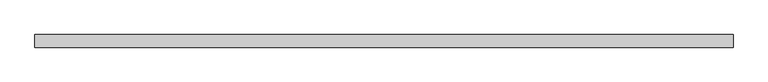
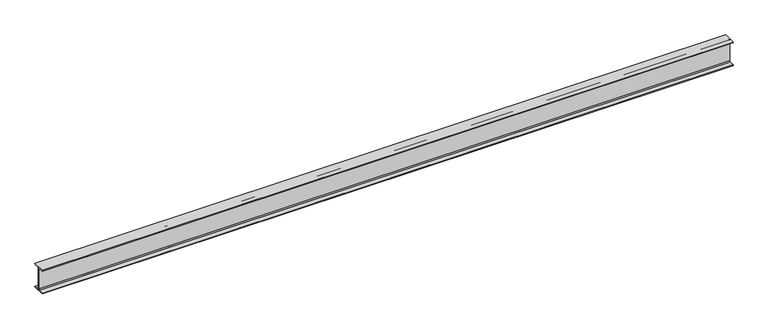
"""IFC4 building model written with IfcOpenShell, lengths in millimetres: beam geometry, 0912_Steel Framing_H-KSD3502 : H_SB_ASB_H-350x175x7x11."""

from ifc_helpers import new_model, si_unit, point, frame, frame_2d, origin, place, context, project, spatial, polyline, circle_curve, trimmed, segment, composite_curve, outline, extrude, source, transform, mapped, element, save


def beam_b0d276df(model_context):
    return source(origin(), model_context, "Body", "SweptSolid", [
        extrude(outline(composite_curve([segment(polyline([(87.5, -164.0), (87.5, -175.0), (-87.5, -175.0), (-87.5, -164.0), (-17.5, -164.0)]), True, "CONTINUOUS"), segment(trimmed(circle_curve(frame_2d((-17.5, -150.0)), 14.0), [point((-17.5, -164.0))], [point((-3.5, -150.0))], True, "CARTESIAN"), True, "CONTINUOUS"), segment(polyline([(-3.5, -150.0), (-3.5, 150.0)]), True, "CONTINUOUS"), segment(trimmed(circle_curve(frame_2d((-17.5, 150.0)), 14.0), [point((-3.5, 150.0))], [point((-17.5, 164.0))], True, "CARTESIAN"), True, "CONTINUOUS"), segment(polyline([(-17.5, 164.0), (-87.5, 164.0), (-87.5, 175.0), (87.5, 175.0), (87.5, 164.0), (17.5, 164.0)]), True, "CONTINUOUS"), segment(trimmed(circle_curve(frame_2d((17.5, 150.0)), 14.0), [point((17.5, 164.0))], [point((3.5, 150.0))], True, "CARTESIAN"), True, "CONTINUOUS"), segment(polyline([(3.5, 150.0), (3.5, -150.0)]), True, "CONTINUOUS"), segment(trimmed(circle_curve(frame_2d((17.5, -150.0)), 14.0), [point((3.5, -150.0))], [point((17.5, -164.0))], True, "CARTESIAN"), True, "CONTINUOUS"), segment(polyline([(17.5, -164.0), (87.5, -164.0)]), True, "CONTINUOUS")], self_intersect=False)), frame((-4837.3, 0.0, 0.0), z_axis=(1.0, 0.0, 0.0), x_axis=(0.0, 1.0, 0.0)), (0.0, 0.0, 1.0), 9699.6),
    ])


if __name__ == "__main__":
    model = new_model("IFC4")
    model_context = context("Model", 3, world=origin())
    ifc_project = project(units=[si_unit("LENGTHUNIT", "METRE", prefix="MILLI")], contexts=[model_context])
    site = spatial("IfcSite", under=ifc_project)
    building = spatial("IfcBuilding", under=site)
    placement = place(None, origin())
    beam_shape = beam_b0d276df(model_context)
    element("IfcBeam", 1, ObjectType="0912_Steel Framing_H-KSD3502 : H_SB_ASB_H-350x175x7x11", at=placement, inside=building, context=model_context, shape_type="MappedRepresentation", body=[
        mapped(beam_shape, transform((0.0, 0.0, 0.0), x_axis=(1.0, 0.0, 0.0), y_axis=(0.0, 1.0, 0.0), z_axis=(0.0, 0.0, 1.0))),
    ])
    save(model, "model.ifc")

# Revit data of these elements
# Type "0912_Steel Framing_H-KSD3502 : H_SB_ASB_H-350x175x7x11"
#   H_WM Code_1 = "S01AA002-00001 | Main Steel Structure Fabrication Work | Shelter/Building | Medium Steel - Standard (90KG/M>Weight≥30KG/M) | Material: (   )"
#   H_WM Code_2 = "S03AA028-00001 | Main Steel Structure Erection Work | Shelter/Building | Medium Steel (90KG/M>Weight≥30KG/M) | Material: (   )"
#   H_WM Code_3 = "S01AA010-00001 | Main Steel Structure Fabrication Work | Shelter/Building | Steel Painting/Coating | for Non-Fireproofed Steel Surface, Surface Preparation, Primer, Second & Final Coat | Material: (   )"
#   H_Q'ty Cal Type Tag = "SB-Q2"
#   Width = 17.5 cm
#   Web Thickness = 0.7 cm
#   Web Fillet = 1.4 cm
#   Warping Constant = 282000.0 cm⁶
#   W = 0
#   Torsional Moment of Inertia = 19.4042 cm⁴
#   Section Area = 63.14 cm²
#   Plastic Modulus weak axis = 174.0 cm³
#   Plastic Modulus strong axis = 868.0 cm³
#   Perimeter = 1.36 m²/m
#   Nominal Weight = 49.60 kgf/m
#   Moment of Inertia weak axis = 984.00 cm⁴
#   Moment of Inertia strong axis = 13600.00 cm⁴
#   Height = 35.0 cm
#   Flange Thickness = 1.1 cm
#   Elastic Modulus weak axis = 112.0 cm³
#   Elastic Modulus strong axis = 775.0 cm³
#   Centroid Vertical = 17.5 cm
#   Centroid Horizontal = 8.75 cm
#   Ix = 136000000
#   Length [instance default] = 1.5240 m
#   Zx = 868000
#   b = 0.1750 m
#   h = 0.3500 m
#   r = 0.0140 m
#   s = 0.0070 m
#   t = 0.0110 m
#   A = 0.006314 m²
#   Structural Material [instance default] = Steel, 45-345
#   Assembly Code = ""
# Element 1 (IfcBeam, "0912_Steel Framing_H-KSD3502 : H_SB_ASB_H-350x175x7x11")
#   Structural Material = none
# Materials
#   "Steel, 45-345": class "Metal", colour RGB 189 187 185, transparency 0, Description = "Steel 345 MPa", Cost = 0
